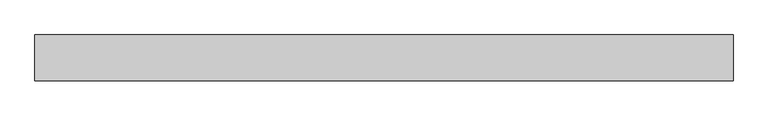
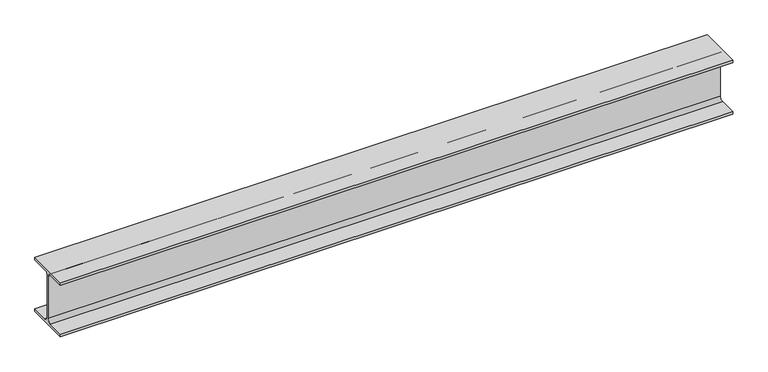
"""IFC4 building model written with IfcOpenShell, lengths in millimetres: beam geometry, 0912_Steel Framing_H-KSD3502 : H_SB_ASB_H-194x150x6x9."""

from ifc_helpers import new_model, si_unit, point, frame, frame_2d, origin, place, context, project, spatial, polyline, circle_curve, trimmed, segment, composite_curve, outline, extrude, source, transform, mapped, element, save


def beam_a62f083a(model_context):
    return source(origin(), model_context, "Body", "SweptSolid", [
        extrude(outline(composite_curve([segment(polyline([(-75.0, -88.0), (-16.0, -88.0)]), True, "CONTINUOUS"), segment(trimmed(circle_curve(frame_2d((-16.0, -75.0)), 13.0), [point((-16.0, -88.0))], [point((-3.0, -75.0))], True, "CARTESIAN"), True, "CONTINUOUS"), segment(polyline([(-3.0, -75.0), (-3.0, 75.0)]), True, "CONTINUOUS"), segment(trimmed(circle_curve(frame_2d((-16.0, 75.0)), 13.0), [point((-3.0, 75.0))], [point((-16.0, 88.0))], True, "CARTESIAN"), True, "CONTINUOUS"), segment(polyline([(-16.0, 88.0), (-75.0, 88.0), (-75.0, 97.0), (75.0, 97.0), (75.0, 88.0), (16.0, 88.0)]), True, "CONTINUOUS"), segment(trimmed(circle_curve(frame_2d((16.0, 75.0)), 13.0), [point((16.0, 88.0))], [point((3.0, 75.0))], True, "CARTESIAN"), True, "CONTINUOUS"), segment(polyline([(3.0, 75.0), (3.0, -75.0)]), True, "CONTINUOUS"), segment(trimmed(circle_curve(frame_2d((16.0, -75.0)), 13.0), [point((3.0, -75.0))], [point((16.0, -88.0))], True, "CARTESIAN"), True, "CONTINUOUS"), segment(polyline([(16.0, -88.0), (75.0, -88.0), (75.0, -97.0), (-75.0, -97.0), (-75.0, -88.0)]), True, "CONTINUOUS")], self_intersect=False)), frame((-700.4863388, 0.0, 0.0), z_axis=(1.0, 0.0, 0.0), x_axis=(0.0, 1.0, 0.0)), (0.0, 0.0, 1.0), 2280.3480504),
    ])


if __name__ == "__main__":
    model = new_model("IFC4")
    model_context = context("Model", 3, world=origin())
    ifc_project = project(units=[si_unit("LENGTHUNIT", "METRE", prefix="MILLI")], contexts=[model_context])
    site = spatial("IfcSite", under=ifc_project)
    building = spatial("IfcBuilding", under=site)
    placement = place(None, origin())
    beam_shape = beam_a62f083a(model_context)
    element("IfcBeam", 1, ObjectType="0912_Steel Framing_H-KSD3502 : H_SB_ASB_H-194x150x6x9", at=placement, inside=building, context=model_context, shape_type="MappedRepresentation", body=[
        mapped(beam_shape, transform((0.0, 0.0, 0.0), x_axis=(1.0, 0.0, 0.0), y_axis=(0.0, 1.0, 0.0), z_axis=(0.0, 0.0, 1.0))),
    ])
    save(model, "model.ifc")

# Revit data of these elements
# Type "0912_Steel Framing_H-KSD3502 : H_SB_ASB_H-194x150x6x9"
#   H_WM Code_1 = "S01AA002-00001 | Main Steel Structure Fabrication Work | Shelter/Building | Medium Steel - Standard (90KG/M>Weight≥30KG/M) | Material: (   )"
#   H_WM Code_2 = "S03AA028-00001 | Main Steel Structure Erection Work | Shelter/Building | Medium Steel (90KG/M>Weight≥30KG/M) | Material: (   )"
#   H_WM Code_3 = "S01AA010-00001 | Main Steel Structure Fabrication Work | Shelter/Building | Steel Painting/Coating | for Non-Fireproofed Steel Surface, Surface Preparation, Primer, Second & Final Coat | Material: (   )"
#   H_Q'ty Cal Type Tag = "SB-Q2"
#   Width = 15.0 cm
#   Web Thickness = 0.6 cm
#   Web Fillet = 1.3 cm
#   Warping Constant = 43316.0 cm⁶
#   W = 0
#   Torsional Moment of Inertia = 8.622 cm⁴
#   Section Area = 39.01 cm²
#   Plastic Modulus weak axis = 104.0 cm³
#   Plastic Modulus strong axis = 309.0 cm³
#   Perimeter = 0.95 m²/m
#   Nominal Weight = 30.60 kgf/m
#   Moment of Inertia weak axis = 507.00 cm⁴
#   Moment of Inertia strong axis = 2690.00 cm⁴
#   Height = 19.4 cm
#   Flange Thickness = 0.9 cm
#   Elastic Modulus weak axis = 67.6 cm³
#   Elastic Modulus strong axis = 277.0 cm³
#   Centroid Vertical = 9.7 cm
#   Centroid Horizontal = 7.5 cm
#   Ix = 26900000
#   Length [instance default] = 1.5240 m
#   Zx = 309000
#   b = 0.1500 m
#   h = 0.1940 m
#   r = 0.0130 m
#   s = 0.0060 m
#   t = 0.0090 m
#   A = 0.003901 m²
#   Structural Material [instance default] = Steel, 45-345
#   Assembly Code = ""
# Element 1 (IfcBeam, "0912_Steel Framing_H-KSD3502 : H_SB_ASB_H-194x150x6x9")
#   Structural Material = none
# Materials
#   "Steel, 45-345": class "Metal", colour RGB 189 187 185, transparency 0, Description = "Steel 345 MPa", Cost = 0
